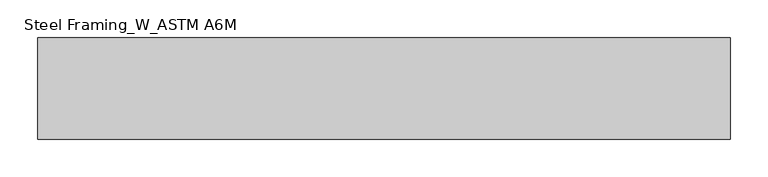
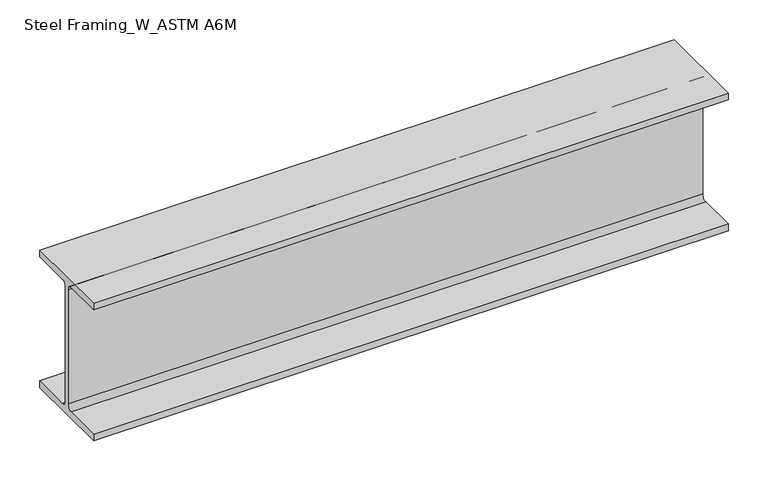
"""IFC4 building model written with IfcOpenShell, lengths in millimetres: beam geometry, Steel Framing_W_ASTM A6M : H_SB_AR_S02_W200x31.3_B6."""

from ifc_helpers import new_model, si_unit, point, frame, frame_2d, origin, place, context, project, spatial, polyline, circle_curve, trimmed, segment, composite_curve, outline, extrude, source, transform, mapped, element, save


def steel_framing_w_astm_a6m_90a0bae4(model_context):
    return source(origin(), model_context, "Body", "SweptSolid", [
        extrude(outline(composite_curve([segment(polyline([(67.0, -94.8), (67.0, -105.0), (-67.0, -105.0), (-67.0, -94.8), (-10.775, -94.8)]), True, "CONTINUOUS"), segment(trimmed(circle_curve(frame_2d((-10.775, -87.2)), 7.6), [point((-10.775, -94.8))], [point((-3.175, -87.2))], True, "CARTESIAN"), True, "CONTINUOUS"), segment(polyline([(-3.175, -87.2), (-3.175, 87.2)]), True, "CONTINUOUS"), segment(trimmed(circle_curve(frame_2d((-10.775, 87.2)), 7.6), [point((-3.175, 87.2))], [point((-10.775, 94.8))], True, "CARTESIAN"), True, "CONTINUOUS"), segment(polyline([(-10.775, 94.8), (-67.0, 94.8), (-67.0, 105.0), (67.0, 105.0), (67.0, 94.8), (10.775, 94.8)]), True, "CONTINUOUS"), segment(trimmed(circle_curve(frame_2d((10.775, 87.2)), 7.6), [point((10.775, 94.8))], [point((3.175, 87.2))], True, "CARTESIAN"), True, "CONTINUOUS"), segment(polyline([(3.175, 87.2), (3.175, -87.2)]), True, "CONTINUOUS"), segment(trimmed(circle_curve(frame_2d((10.775, -87.2)), 7.6), [point((3.175, -87.2))], [point((10.775, -94.8))], True, "CARTESIAN"), True, "CONTINUOUS"), segment(polyline([(10.775, -94.8), (67.0, -94.8)]), True, "CONTINUOUS")], self_intersect=False)), frame((-421.3, 0.0, 0.0), z_axis=(1.0, 0.0, 0.0), x_axis=(0.0, 1.0, 0.0)), (0.0, 0.0, 1.0), 916.6),
    ])


if __name__ == "__main__":
    model = new_model("IFC4")
    model_context = context("Model", 3, world=origin())
    ifc_project = project(units=[si_unit("LENGTHUNIT", "METRE", prefix="MILLI")], contexts=[model_context])
    site = spatial("IfcSite", under=ifc_project)
    building = spatial("IfcBuilding", under=site)
    placement = place(None, origin())
    steel_framing_w_astm_a6m_shape = steel_framing_w_astm_a6m_90a0bae4(model_context)
    element("IfcBeam", 1, ObjectType="Steel Framing_W_ASTM A6M : H_SB_AR_S02_W200x31.3_B6", at=placement, inside=building, context=model_context, shape_type="MappedRepresentation", body=[
        mapped(steel_framing_w_astm_a6m_shape, transform((0.0, 0.0, 0.0), x_axis=(1.0, 0.0, 0.0), y_axis=(0.0, 1.0, 0.0), z_axis=(0.0, 0.0, 1.0))),
    ])
    save(model, "model.ifc")

# Revit data of these elements
# Type "Steel Framing_W_ASTM A6M : H_SB_AR_S02_W200x31.3_B6"
#   Type Mark = "B6"
#   Section Name Key = "W8x21"
#   Width = 13.4 cm
#   Web Thickness = 0.635 cm
#   Web Fillet = 0.76 cm
#   Warping Constant = 40800.0 cm⁶
#   Torsional Moment of Inertia = 11.70 cm⁴
#   Section Area = 39.7 cm²
#   Plastic Modulus weak axis = 93.2 cm³
#   Plastic Modulus strong axis = 334.0 cm³
#   Perimeter = 0.93 m²/m
#   Nominal Weight = 31.30 kgf/m
#   Moment of Inertia weak axis = 407.00 cm⁴
#   Moment of Inertia strong axis = 3130.00 cm⁴
#   Height = 21.0 cm
#   Flange Thickness = 1.02 cm
#   Elastic Modulus weak axis = 60.8 cm³
#   Elastic Modulus strong axis = 298.0 cm³
#   Centroid Vertical = 10.5 cm
#   Centroid Horizontal = 6.7 cm
#   Length [instance default] = 1500 mm
#   Structural Material [instance default] = Steel, 45-345
#   Bolt Spacing = 0
#   Assembly Code = ""
# Element 1 (IfcBeam, "Steel Framing_W_ASTM A6M : H_SB_AR_S02_W200x31.3_B6")
#   Materials on its faces: "Steel, 45-345"
# Materials
#   "Steel, 45-345": class "Metal", colour RGB 189 187 185, transparency 0, Description = "Steel 345 MPa", Cost = 0
